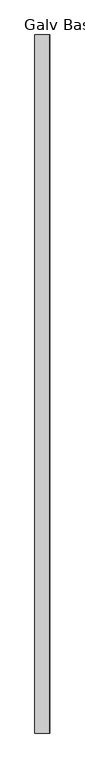
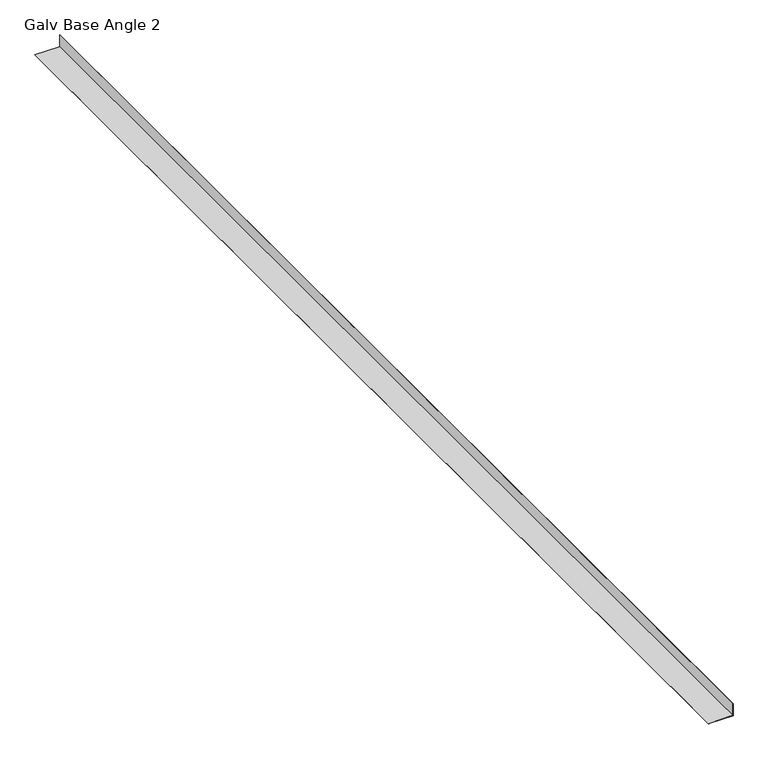
"""IFC4 building model written with IfcOpenShell, lengths in millimetres: proxy geometry, Galv Base Angle 2 : CF Galv L 4x2x16ga."""

from ifc_helpers import new_model, si_unit, frame, origin, place, context, project, spatial, polyline, outline, extrude, source, transform, mapped, element, save


def galv_base_angle_2_de8a329e(model_context):
    return source(origin(), model_context, "Body", "SweptSolid", [
        extrude(outline(polyline([(0.93726, 590250.3936739), (0.0, 590250.3936739), (0.0, 590351.9936739), (50.8, 590351.9936739), (50.8, 590351.0564139), (0.93726, 590351.0564139), (0.93726, 590250.3936739)])), frame((0.0, -536417.5913841, 0.0), z_axis=(0.0, 1.0, 0.0), x_axis=(0.0, 0.0, 1.0)), (0.0, 0.0, 1.0), 4743.45),
    ])


if __name__ == "__main__":
    model = new_model("IFC4")
    model_context = context("Model", 3, world=origin())
    ifc_project = project(units=[si_unit("LENGTHUNIT", "METRE", prefix="MILLI")], contexts=[model_context])
    site = spatial("IfcSite", under=ifc_project)
    building = spatial("IfcBuilding", under=site)
    placement = place(None, origin())
    galv_base_angle_2_shape = galv_base_angle_2_de8a329e(model_context)
    element("IfcBuildingElementProxy", 1, Name="Galv Base Angle 2 : CF Galv L 4x2x16ga", ObjectType="Galv Base Angle 2 : CF Galv L 4x2x16ga", at=placement, inside=building, context=model_context, shape_type="MappedRepresentation", body=[
        mapped(galv_base_angle_2_shape, transform((0.0, 0.0, 0.0), x_axis=(1.0, 0.0, 0.0), y_axis=(0.0, 1.0, 0.0), z_axis=(0.0, 0.0, 1.0))),
    ])
    save(model, "model.ifc")

# Revit data of these elements
# Element 1 (IfcBuildingElementProxy, "Galv Base Angle 2 : CF Galv L 4x2x16ga")
#   Materials on its faces: "4\"X2\" L - COLD-FORMED GALV."
# Materials
#   "4\"X2\" L - COLD-FORMED GALV.": class "Generic", colour RGB 143 142 141, transparency 0, Cost = 0
